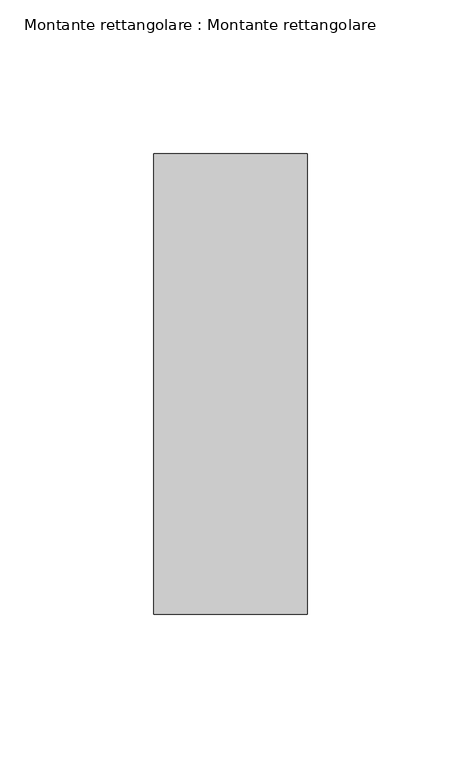
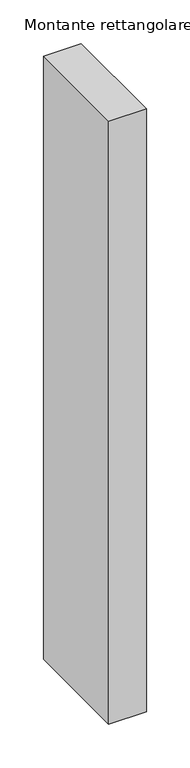
"""IFC4 building model written with IfcOpenShell, lengths in millimetres: member geometry, Montante rettangolare : Montante rettangolare."""

from ifc_helpers import new_model, si_unit, frame, origin, place, context, project, spatial, polyline, outline, extrude, source, transform, mapped, element, save


def montante_rettangolare_montante_rettangolare_3e62889d(model_context):
    return source(origin(), model_context, "Body", "SweptSolid", [
        extrude(outline(polyline([(0.0, 75.0), (0.0, -75.0), (-50.0, -75.0), (-50.0, 75.0), (0.0, 75.0)])), frame((0.0, 0.0, -845.0), z_axis=(0.0, 0.0, 1.0), x_axis=(1.0, 0.0, 0.0)), (0.0, 0.0, 1.0), 845.0),
    ])


if __name__ == "__main__":
    model = new_model("IFC4")
    model_context = context("Model", 3, world=origin())
    ifc_project = project(units=[si_unit("LENGTHUNIT", "METRE", prefix="MILLI")], contexts=[model_context])
    site = spatial("IfcSite", under=ifc_project)
    building = spatial("IfcBuilding", under=site)
    placement = place(None, origin())
    montante_rettangolare_montante_rettangolare_shape = montante_rettangolare_montante_rettangolare_3e62889d(model_context)
    element("IfcMember", 1, ObjectType="Montante rettangolare : Montante rettangolare", at=placement, inside=building, context=model_context, shape_type="MappedRepresentation", body=[
        mapped(montante_rettangolare_montante_rettangolare_shape, transform((0.0, 0.0, 0.0), x_axis=(1.0, 0.0, 0.0), y_axis=(0.0, 1.0, 0.0), z_axis=(0.0, 0.0, 1.0))),
    ])
    save(model, "model.ifc")

# Revit data of these elements
# Type "Montante rettangolare : Montante rettangolare"
#   built-in parameter 1007304 = 0.492126 (stored number, unit not read)
#   built-in parameter 1007301 = 0.082021 (stored number, unit not read)
#   built-in parameter 1007300 = 0.082021 (stored number, unit not read)
# Element 1 (IfcMember, "Montante rettangolare : Montante rettangolare")
#   Materials on its faces: "Acciaio"
# Materials
#   "Acciaio": class "Metallo", colour RGB 247 247 247, transparency 0, Description = "Acciaio, finitura zigrinata", Cost = 0
